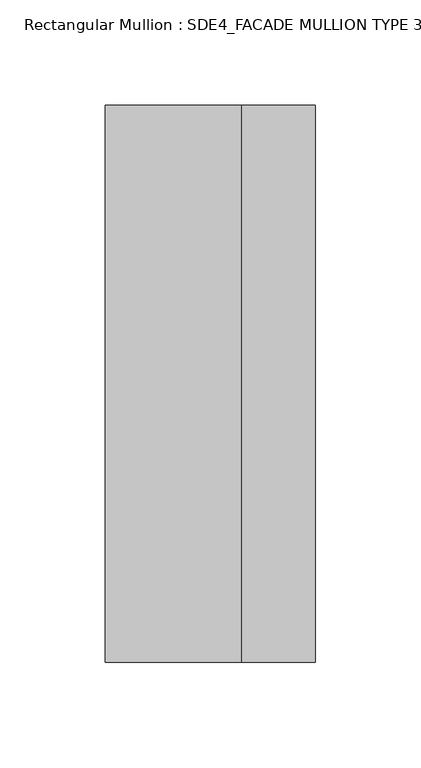
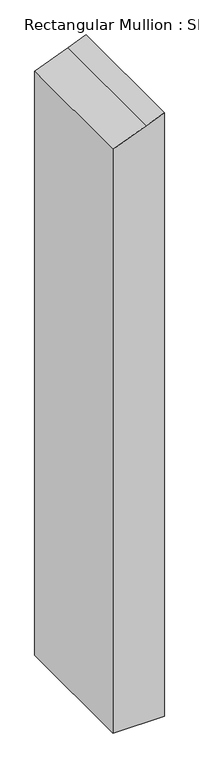
"""IFC4 building model written with IfcOpenShell, lengths in millimetres: member geometry, Rectangular Mullion : SDE4_FACADE MULLION TYPE 3."""

from ifc_helpers import new_model, si_unit, frame, origin, place, context, project, spatial, polyline, outline, extrude, source, transform, mapped, element, save


def rectangular_mullion_sde4_facade_mullion_type_3_504cdb45(model_context):
    return source(origin(), model_context, "Body", "SweptSolid", [
        extrude(outline(polyline([(-23.0813185, 50.0), (-37.1390676, 14.8556271), (-63.0813185, -50.0), (-1267.974544, -50.0), (-1267.974544, 50.0), (-23.0813185, 50.0)])), frame((0.0, -132.5, 0.0), z_axis=(0.0, 1.0, 0.0), x_axis=(0.0, 0.0, 1.0)), (0.0, 0.0, 1.0), 265.0),
    ])


if __name__ == "__main__":
    model = new_model("IFC4")
    model_context = context("Model", 3, world=origin())
    ifc_project = project(units=[si_unit("LENGTHUNIT", "METRE", prefix="MILLI")], contexts=[model_context])
    site = spatial("IfcSite", under=ifc_project)
    building = spatial("IfcBuilding", under=site)
    placement = place(None, origin())
    rectangular_mullion_sde4_facade_mullion_type_3_shape = rectangular_mullion_sde4_facade_mullion_type_3_504cdb45(model_context)
    element("IfcMember", 1, ObjectType="Rectangular Mullion : SDE4_FACADE MULLION TYPE 3", at=placement, inside=building, context=model_context, shape_type="MappedRepresentation", body=[
        mapped(rectangular_mullion_sde4_facade_mullion_type_3_shape, transform((0.0, 0.0, 0.0), x_axis=(1.0, 0.0, 0.0), y_axis=(0.0, 1.0, 0.0), z_axis=(0.0, 0.0, 1.0))),
    ])
    save(model, "model.ifc")

# Revit data of these elements
# Type "Rectangular Mullion : SDE4_FACADE MULLION TYPE 3"
#   built-in parameter 1007322 = 0.869423 (stored number, unit not read)
#   built-in parameter 1007321 = 0.164042 (stored number, unit not read)
#   built-in parameter 1007320 = 0.164042 (stored number, unit not read)
